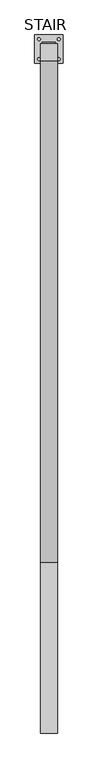
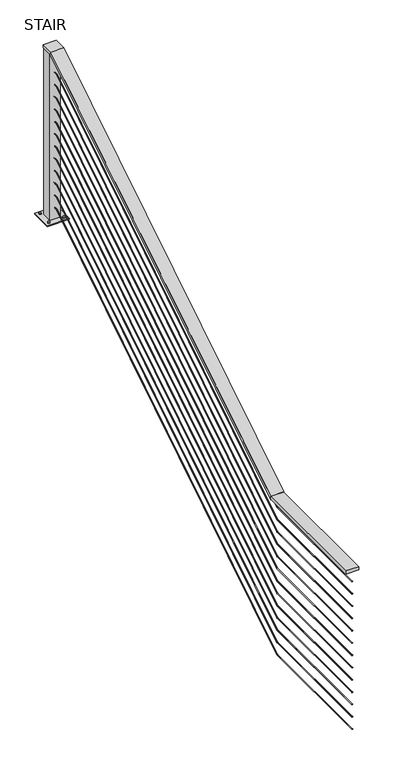
"""IFC4 building model written with IfcOpenShell, lengths in millimetres: railing geometry, STAIR."""

from ifc_helpers import new_model, si_unit, point, frame, frame_2d, origin, place, context, project, spatial, polyline, circle_curve, ellipse_curve, trimmed, segment, composite_curve, outline, extrude, faceted_brep, source, transform, mapped, element, save
from ifc_brep_helpers import plane_surface, cylinder_surface, advanced_brep


def stair_1ed1dee3(model_context):
    return source(origin(), model_context, "Body", "SolidModel", [
        faceted_brep([(26115.1620052, 2826.8043237, 2466.975), (26038.9620052, 2826.8043237, 2466.975), (26038.9620052, 2826.8043237, 2447.925), (26115.1620052, 2826.8043237, 2447.925), (26115.1620052, 3588.8043237, 2466.975), (26115.1620052, 3588.8043237, 2447.925), (26038.9620052, 3588.8043237, 2447.925), (26038.9620052, 3588.8043237, 2466.975)], [[[0, 1, 2, 3]], [[4, 5, 6, 7]], [[1, 0, 4, 7]], [[2, 1, 7, 6]], [[3, 2, 6, 5]], [[0, 3, 5, 4]]]),
        faceted_brep([(26115.1620052, 3588.8043237, 2468.6895104), (26038.9620052, 3588.8043237, 2468.6895104), (26038.9620052, 3588.8043237, 2446.2104896), (26115.1620052, 3588.8043237, 2446.2104896), (26115.1620052, 5821.2673274, 3867.15), (26038.9620052, 5821.2673274, 3867.15), (26038.9620052, 5826.7413199, 3848.1), (26115.1620052, 5826.7413199, 3848.1), (26115.1620052, 5898.8634079, 3867.15), (26115.1620052, 5898.8634079, 3848.1), (26038.9620052, 5898.8634079, 3848.1), (26038.9620052, 5898.8634079, 3867.15)], [[[0, 1, 2, 3]], [[1, 0, 4, 5]], [[2, 1, 5, 6]], [[3, 2, 6, 7]], [[0, 3, 7, 4]], [[8, 9, 10, 11]], [[5, 4, 8, 11]], [[6, 5, 11, 10]], [[7, 6, 10, 9]], [[4, 7, 9, 8]]]),
        advanced_brep(
        [(26074.6807552, 2826.8043237, 2388.39375), (26079.4432552, 2826.8043237, 2388.39375), (26074.6807552, 3588.8043237, 2388.39375), (26079.4432552, 3588.8043237, 2388.39375)],
        [
            (0, 1, circle_curve(frame((26077.0620052, 2826.8043237, 2388.39375), z_axis=(0.0, -1.0, 0.0), x_axis=(1.0, 0.0, 0.0)), 2.38125)),
            (1, 0, circle_curve(frame((26077.0620052, 2826.8043237, 2388.39375), z_axis=(0.0, -1.0, 0.0), x_axis=(1.0, 0.0, 0.0)), 2.38125)),
            (2, 3, circle_curve(frame((26077.0620052, 3588.8043237, 2388.39375), z_axis=(0.0, 1.0, 0.0), x_axis=(1.0, 0.0, 0.0)), 2.38125)),
            (3, 2, circle_curve(frame((26077.0620052, 3588.8043237, 2388.39375), z_axis=(0.0, 1.0, 0.0), x_axis=(1.0, 0.0, 0.0)), 2.38125)),
            (0, 2),
            (3, 1),
        ],
        [
            plane_surface(frame((26077.0620052, 2826.8043237, 2390.775), z_axis=(0.0, -1.0, 0.0), x_axis=(0.0, 0.0, 1.0))),
            plane_surface(frame((26077.0620052, 3588.8043237, 2390.775), z_axis=(0.0, 1.0, 0.0), x_axis=(0.0, 0.0, 1.0))),
            cylinder_surface(frame((26077.0620052, 2826.8043237, 2388.39375), z_axis=(0.0, -1.0, 0.0), x_axis=(1.0, 0.0, 0.0)), 2.38125),
        ],
        [
            (0, [[1, 2]]),
            (1, [[3, 4]]),
            (2, [[-1, 5, -4, 6]]),
            (2, [[-2, -6, -3, -5]]),
        ],
    ),
        advanced_brep(
        [(26074.6807552, 3588.8043237, 2387.9651224), (26079.4432552, 3588.8043237, 2387.9651224), (26074.6807552, 5824.6885727, 3788.56875), (26079.4432552, 5824.6885727, 3788.56875), (26074.6807552, 5898.8634079, 3788.56875), (26079.4432552, 5898.8634079, 3788.56875)],
        [
            (0, 1, ellipse_curve(frame((26077.0620052, 3588.8043237, 2387.9651224), z_axis=(0.0, -1.0, 0.0), x_axis=(0.0, 0.0, -1.0)), 2.8098776, 2.38125)),
            (1, 0, ellipse_curve(frame((26077.0620052, 3588.8043237, 2387.9651224), z_axis=(0.0, -1.0, 0.0), x_axis=(0.0, 0.0, -1.0)), 2.8098776, 2.38125)),
            (0, 2),
            (2, 3, ellipse_curve(frame((26077.0620052, 5824.6885727, 3788.56875), z_axis=(0.0, -0.9611079128273462, -0.2761730977134852), x_axis=(0.0, 0.27617309771348514, -0.9611079128273461)), 2.4776094, 2.38125)),
            (3, 1),
            (3, 2, ellipse_curve(frame((26077.0620052, 5824.6885727, 3788.56875), z_axis=(0.0, -0.9611079128273462, -0.2761730977134852), x_axis=(0.0, 0.27617309771348514, -0.9611079128273461)), 2.4776094, 2.38125)),
            (4, 5, circle_curve(frame((26077.0620052, 5898.8634079, 3788.56875), z_axis=(0.0, 1.0, 0.0), x_axis=(1.0, 0.0, 0.0)), 2.38125)),
            (5, 4, circle_curve(frame((26077.0620052, 5898.8634079, 3788.56875), z_axis=(0.0, 1.0, 0.0), x_axis=(1.0, 0.0, 0.0)), 2.38125)),
            (2, 4),
            (5, 3),
        ],
        [
            plane_surface(frame((26077.0620052, 3588.8043237, 2390.775), z_axis=(0.0, -1.0, 0.0), x_axis=(0.0, 0.0, 1.0))),
            cylinder_surface(frame((26077.0620052, 3590.0684443, 2388.7569934), z_axis=(0.0, -0.8474568401986755, -0.530864299044941), x_axis=(1.0, 0.0, 0.0)), 2.38125),
            plane_surface(frame((26077.0620052, 5898.8634079, 3790.95), z_axis=(0.0, 1.0, 0.0), x_axis=(0.0, 0.0, 1.0))),
            cylinder_surface(frame((26077.0620052, 5824.0043237, 3788.56875), z_axis=(0.0, -1.0, 0.0), x_axis=(1.0, 0.0, 0.0)), 2.38125),
        ],
        [
            (0, [[1, 2]]),
            (1, [[-1, 3, 4, 5]]),
            (1, [[-2, -5, 6, -3]]),
            (2, [[7, 8]]),
            (3, [[-4, 9, -8, 10]]),
            (3, [[-6, -10, -7, -9]]),
        ],
    ),
        advanced_brep(
        [(26074.6807552, 2826.8043237, 2312.19375), (26079.4432552, 2826.8043237, 2312.19375), (26074.6807552, 3588.8043237, 2312.19375), (26079.4432552, 3588.8043237, 2312.19375)],
        [
            (0, 1, circle_curve(frame((26077.0620052, 2826.8043237, 2312.19375), z_axis=(0.0, -1.0, 0.0), x_axis=(1.0, 0.0, 0.0)), 2.38125)),
            (1, 0, circle_curve(frame((26077.0620052, 2826.8043237, 2312.19375), z_axis=(0.0, -1.0, 0.0), x_axis=(1.0, 0.0, 0.0)), 2.38125)),
            (2, 3, circle_curve(frame((26077.0620052, 3588.8043237, 2312.19375), z_axis=(0.0, 1.0, 0.0), x_axis=(1.0, 0.0, 0.0)), 2.38125)),
            (3, 2, circle_curve(frame((26077.0620052, 3588.8043237, 2312.19375), z_axis=(0.0, 1.0, 0.0), x_axis=(1.0, 0.0, 0.0)), 2.38125)),
            (0, 2),
            (3, 1),
        ],
        [
            plane_surface(frame((26077.0620052, 2826.8043237, 2314.575), z_axis=(0.0, -1.0, 0.0), x_axis=(0.0, 0.0, 1.0))),
            plane_surface(frame((26077.0620052, 3588.8043237, 2314.575), z_axis=(0.0, 1.0, 0.0), x_axis=(0.0, 0.0, 1.0))),
            cylinder_surface(frame((26077.0620052, 2826.8043237, 2312.19375), z_axis=(0.0, -1.0, 0.0), x_axis=(1.0, 0.0, 0.0)), 2.38125),
        ],
        [
            (0, [[1, 2]]),
            (1, [[3, 4]]),
            (2, [[-1, 5, -4, 6]]),
            (2, [[-2, -6, -3, -5]]),
        ],
    ),
        advanced_brep(
        [(26074.6807552, 3588.8043237, 2311.7651224), (26079.4432552, 3588.8043237, 2311.7651224), (26074.6807552, 5824.6885727, 3712.36875), (26079.4432552, 5824.6885727, 3712.36875), (26074.6807552, 5898.8634079, 3712.36875), (26079.4432552, 5898.8634079, 3712.36875)],
        [
            (0, 1, ellipse_curve(frame((26077.0620052, 3588.8043237, 2311.7651224), z_axis=(0.0, -1.0, 0.0), x_axis=(0.0, 0.0, -1.0)), 2.8098776, 2.38125)),
            (1, 0, ellipse_curve(frame((26077.0620052, 3588.8043237, 2311.7651224), z_axis=(0.0, -1.0, 0.0), x_axis=(0.0, 0.0, -1.0)), 2.8098776, 2.38125)),
            (0, 2),
            (2, 3, ellipse_curve(frame((26077.0620052, 5824.6885727, 3712.36875), z_axis=(0.0, -0.9611079128273462, -0.2761730977134852), x_axis=(0.0, 0.27617309771348514, -0.9611079128273461)), 2.4776094, 2.38125)),
            (3, 1),
            (3, 2, ellipse_curve(frame((26077.0620052, 5824.6885727, 3712.36875), z_axis=(0.0, -0.9611079128273462, -0.2761730977134852), x_axis=(0.0, 0.27617309771348514, -0.9611079128273461)), 2.4776094, 2.38125)),
            (4, 5, circle_curve(frame((26077.0620052, 5898.8634079, 3712.36875), z_axis=(0.0, 1.0, 0.0), x_axis=(1.0, 0.0, 0.0)), 2.38125)),
            (5, 4, circle_curve(frame((26077.0620052, 5898.8634079, 3712.36875), z_axis=(0.0, 1.0, 0.0), x_axis=(1.0, 0.0, 0.0)), 2.38125)),
            (2, 4),
            (5, 3),
        ],
        [
            plane_surface(frame((26077.0620052, 3588.8043237, 2314.575), z_axis=(0.0, -1.0, 0.0), x_axis=(0.0, 0.0, 1.0))),
            cylinder_surface(frame((26077.0620052, 3590.0684443, 2312.5569934), z_axis=(0.0, -0.8474568401986755, -0.530864299044941), x_axis=(1.0, 0.0, 0.0)), 2.38125),
            plane_surface(frame((26077.0620052, 5898.8634079, 3714.75), z_axis=(0.0, 1.0, 0.0), x_axis=(0.0, 0.0, 1.0))),
            cylinder_surface(frame((26077.0620052, 5824.0043237, 3712.36875), z_axis=(0.0, -1.0, 0.0), x_axis=(1.0, 0.0, 0.0)), 2.38125),
        ],
        [
            (0, [[1, 2]]),
            (1, [[-1, 3, 4, 5]]),
            (1, [[-2, -5, 6, -3]]),
            (2, [[7, 8]]),
            (3, [[-4, 9, -8, 10]]),
            (3, [[-6, -10, -7, -9]]),
        ],
    ),
        advanced_brep(
        [(26074.6807552, 2826.8043237, 2235.99375), (26079.4432552, 2826.8043237, 2235.99375), (26074.6807552, 3588.8043237, 2235.99375), (26079.4432552, 3588.8043237, 2235.99375)],
        [
            (0, 1, circle_curve(frame((26077.0620052, 2826.8043237, 2235.99375), z_axis=(0.0, -1.0, 0.0), x_axis=(1.0, 0.0, 0.0)), 2.38125)),
            (1, 0, circle_curve(frame((26077.0620052, 2826.8043237, 2235.99375), z_axis=(0.0, -1.0, 0.0), x_axis=(1.0, 0.0, 0.0)), 2.38125)),
            (2, 3, circle_curve(frame((26077.0620052, 3588.8043237, 2235.99375), z_axis=(0.0, 1.0, 0.0), x_axis=(1.0, 0.0, 0.0)), 2.38125)),
            (3, 2, circle_curve(frame((26077.0620052, 3588.8043237, 2235.99375), z_axis=(0.0, 1.0, 0.0), x_axis=(1.0, 0.0, 0.0)), 2.38125)),
            (0, 2),
            (3, 1),
        ],
        [
            plane_surface(frame((26077.0620052, 2826.8043237, 2238.375), z_axis=(0.0, -1.0, 0.0), x_axis=(0.0, 0.0, 1.0))),
            plane_surface(frame((26077.0620052, 3588.8043237, 2238.375), z_axis=(0.0, 1.0, 0.0), x_axis=(0.0, 0.0, 1.0))),
            cylinder_surface(frame((26077.0620052, 2826.8043237, 2235.99375), z_axis=(0.0, -1.0, 0.0), x_axis=(1.0, 0.0, 0.0)), 2.38125),
        ],
        [
            (0, [[1, 2]]),
            (1, [[3, 4]]),
            (2, [[-1, 5, -4, 6]]),
            (2, [[-2, -6, -3, -5]]),
        ],
    ),
        advanced_brep(
        [(26074.6807552, 3588.8043237, 2235.5651224), (26079.4432552, 3588.8043237, 2235.5651224), (26074.6807552, 5824.6885727, 3636.16875), (26079.4432552, 5824.6885727, 3636.16875), (26074.6807552, 5898.8634079, 3636.16875), (26079.4432552, 5898.8634079, 3636.16875)],
        [
            (0, 1, ellipse_curve(frame((26077.0620052, 3588.8043237, 2235.5651224), z_axis=(0.0, -1.0, 0.0), x_axis=(0.0, 0.0, -1.0)), 2.8098776, 2.38125)),
            (1, 0, ellipse_curve(frame((26077.0620052, 3588.8043237, 2235.5651224), z_axis=(0.0, -1.0, 0.0), x_axis=(0.0, 0.0, -1.0)), 2.8098776, 2.38125)),
            (0, 2),
            (2, 3, ellipse_curve(frame((26077.0620052, 5824.6885727, 3636.16875), z_axis=(0.0, -0.9611079128273462, -0.2761730977134852), x_axis=(0.0, 0.27617309771348514, -0.9611079128273461)), 2.4776094, 2.38125)),
            (3, 1),
            (3, 2, ellipse_curve(frame((26077.0620052, 5824.6885727, 3636.16875), z_axis=(0.0, -0.9611079128273462, -0.2761730977134852), x_axis=(0.0, 0.27617309771348514, -0.9611079128273461)), 2.4776094, 2.38125)),
            (4, 5, circle_curve(frame((26077.0620052, 5898.8634079, 3636.16875), z_axis=(0.0, 1.0, 0.0), x_axis=(1.0, 0.0, 0.0)), 2.38125)),
            (5, 4, circle_curve(frame((26077.0620052, 5898.8634079, 3636.16875), z_axis=(0.0, 1.0, 0.0), x_axis=(1.0, 0.0, 0.0)), 2.38125)),
            (2, 4),
            (5, 3),
        ],
        [
            plane_surface(frame((26077.0620052, 3588.8043237, 2238.375), z_axis=(0.0, -1.0, 0.0), x_axis=(0.0, 0.0, 1.0))),
            cylinder_surface(frame((26077.0620052, 3590.0684443, 2236.3569934), z_axis=(0.0, -0.8474568401986755, -0.530864299044941), x_axis=(1.0, 0.0, 0.0)), 2.38125),
            plane_surface(frame((26077.0620052, 5898.8634079, 3638.55), z_axis=(0.0, 1.0, 0.0), x_axis=(0.0, 0.0, 1.0))),
            cylinder_surface(frame((26077.0620052, 5824.0043237, 3636.16875), z_axis=(0.0, -1.0, 0.0), x_axis=(1.0, 0.0, 0.0)), 2.38125),
        ],
        [
            (0, [[1, 2]]),
            (1, [[-1, 3, 4, 5]]),
            (1, [[-2, -5, 6, -3]]),
            (2, [[7, 8]]),
            (3, [[-4, 9, -8, 10]]),
            (3, [[-6, -10, -7, -9]]),
        ],
    ),
        advanced_brep(
        [(26074.6807552, 2826.8043237, 2159.79375), (26079.4432552, 2826.8043237, 2159.79375), (26074.6807552, 3588.8043237, 2159.79375), (26079.4432552, 3588.8043237, 2159.79375)],
        [
            (0, 1, circle_curve(frame((26077.0620052, 2826.8043237, 2159.79375), z_axis=(0.0, -1.0, 0.0), x_axis=(1.0, 0.0, 0.0)), 2.38125)),
            (1, 0, circle_curve(frame((26077.0620052, 2826.8043237, 2159.79375), z_axis=(0.0, -1.0, 0.0), x_axis=(1.0, 0.0, 0.0)), 2.38125)),
            (2, 3, circle_curve(frame((26077.0620052, 3588.8043237, 2159.79375), z_axis=(0.0, 1.0, 0.0), x_axis=(1.0, 0.0, 0.0)), 2.38125)),
            (3, 2, circle_curve(frame((26077.0620052, 3588.8043237, 2159.79375), z_axis=(0.0, 1.0, 0.0), x_axis=(1.0, 0.0, 0.0)), 2.38125)),
            (0, 2),
            (3, 1),
        ],
        [
            plane_surface(frame((26077.0620052, 2826.8043237, 2162.175), z_axis=(0.0, -1.0, 0.0), x_axis=(0.0, 0.0, 1.0))),
            plane_surface(frame((26077.0620052, 3588.8043237, 2162.175), z_axis=(0.0, 1.0, 0.0), x_axis=(0.0, 0.0, 1.0))),
            cylinder_surface(frame((26077.0620052, 2826.8043237, 2159.79375), z_axis=(0.0, -1.0, 0.0), x_axis=(1.0, 0.0, 0.0)), 2.38125),
        ],
        [
            (0, [[1, 2]]),
            (1, [[3, 4]]),
            (2, [[-1, 5, -4, 6]]),
            (2, [[-2, -6, -3, -5]]),
        ],
    ),
        advanced_brep(
        [(26074.6807552, 3588.8043237, 2159.3651224), (26079.4432552, 3588.8043237, 2159.3651224), (26074.6807552, 5824.6885727, 3559.96875), (26079.4432552, 5824.6885727, 3559.96875), (26074.6807552, 5898.8634079, 3559.96875), (26079.4432552, 5898.8634079, 3559.96875)],
        [
            (0, 1, ellipse_curve(frame((26077.0620052, 3588.8043237, 2159.3651224), z_axis=(0.0, -1.0, 0.0), x_axis=(0.0, 0.0, -1.0)), 2.8098776, 2.38125)),
            (1, 0, ellipse_curve(frame((26077.0620052, 3588.8043237, 2159.3651224), z_axis=(0.0, -1.0, 0.0), x_axis=(0.0, 0.0, -1.0)), 2.8098776, 2.38125)),
            (0, 2),
            (2, 3, ellipse_curve(frame((26077.0620052, 5824.6885727, 3559.96875), z_axis=(0.0, -0.9611079128273462, -0.2761730977134852), x_axis=(0.0, 0.27617309771348514, -0.9611079128273461)), 2.4776094, 2.38125)),
            (3, 1),
            (3, 2, ellipse_curve(frame((26077.0620052, 5824.6885727, 3559.96875), z_axis=(0.0, -0.9611079128273462, -0.2761730977134852), x_axis=(0.0, 0.27617309771348514, -0.9611079128273461)), 2.4776094, 2.38125)),
            (4, 5, circle_curve(frame((26077.0620052, 5898.8634079, 3559.96875), z_axis=(0.0, 1.0, 0.0), x_axis=(1.0, 0.0, 0.0)), 2.38125)),
            (5, 4, circle_curve(frame((26077.0620052, 5898.8634079, 3559.96875), z_axis=(0.0, 1.0, 0.0), x_axis=(1.0, 0.0, 0.0)), 2.38125)),
            (2, 4),
            (5, 3),
        ],
        [
            plane_surface(frame((26077.0620052, 3588.8043237, 2162.175), z_axis=(0.0, -1.0, 0.0), x_axis=(0.0, 0.0, 1.0))),
            cylinder_surface(frame((26077.0620052, 3590.0684443, 2160.1569934), z_axis=(0.0, -0.8474568401986755, -0.530864299044941), x_axis=(1.0, 0.0, 0.0)), 2.38125),
            plane_surface(frame((26077.0620052, 5898.8634079, 3562.35), z_axis=(0.0, 1.0, 0.0), x_axis=(0.0, 0.0, 1.0))),
            cylinder_surface(frame((26077.0620052, 5824.0043237, 3559.96875), z_axis=(0.0, -1.0, 0.0), x_axis=(1.0, 0.0, 0.0)), 2.38125),
        ],
        [
            (0, [[1, 2]]),
            (1, [[-1, 3, 4, 5]]),
            (1, [[-2, -5, 6, -3]]),
            (2, [[7, 8]]),
            (3, [[-4, 9, -8, 10]]),
            (3, [[-6, -10, -7, -9]]),
        ],
    ),
        advanced_brep(
        [(26074.6807552, 2826.8043237, 2083.59375), (26079.4432552, 2826.8043237, 2083.59375), (26074.6807552, 3588.8043237, 2083.59375), (26079.4432552, 3588.8043237, 2083.59375)],
        [
            (0, 1, circle_curve(frame((26077.0620052, 2826.8043237, 2083.59375), z_axis=(0.0, -1.0, 0.0), x_axis=(1.0, 0.0, 0.0)), 2.38125)),
            (1, 0, circle_curve(frame((26077.0620052, 2826.8043237, 2083.59375), z_axis=(0.0, -1.0, 0.0), x_axis=(1.0, 0.0, 0.0)), 2.38125)),
            (2, 3, circle_curve(frame((26077.0620052, 3588.8043237, 2083.59375), z_axis=(0.0, 1.0, 0.0), x_axis=(1.0, 0.0, 0.0)), 2.38125)),
            (3, 2, circle_curve(frame((26077.0620052, 3588.8043237, 2083.59375), z_axis=(0.0, 1.0, 0.0), x_axis=(1.0, 0.0, 0.0)), 2.38125)),
            (0, 2),
            (3, 1),
        ],
        [
            plane_surface(frame((26077.0620052, 2826.8043237, 2085.975), z_axis=(0.0, -1.0, 0.0), x_axis=(0.0, 0.0, 1.0))),
            plane_surface(frame((26077.0620052, 3588.8043237, 2085.975), z_axis=(0.0, 1.0, 0.0), x_axis=(0.0, 0.0, 1.0))),
            cylinder_surface(frame((26077.0620052, 2826.8043237, 2083.59375), z_axis=(0.0, -1.0, 0.0), x_axis=(1.0, 0.0, 0.0)), 2.38125),
        ],
        [
            (0, [[1, 2]]),
            (1, [[3, 4]]),
            (2, [[-1, 5, -4, 6]]),
            (2, [[-2, -6, -3, -5]]),
        ],
    ),
        advanced_brep(
        [(26074.6807552, 3588.8043237, 2083.1651224), (26079.4432552, 3588.8043237, 2083.1651224), (26074.6807552, 5824.6885727, 3483.76875), (26079.4432552, 5824.6885727, 3483.76875), (26074.6807552, 5898.8634079, 3483.76875), (26079.4432552, 5898.8634079, 3483.76875)],
        [
            (0, 1, ellipse_curve(frame((26077.0620052, 3588.8043237, 2083.1651224), z_axis=(0.0, -1.0, 0.0), x_axis=(0.0, 0.0, -1.0)), 2.8098776, 2.38125)),
            (1, 0, ellipse_curve(frame((26077.0620052, 3588.8043237, 2083.1651224), z_axis=(0.0, -1.0, 0.0), x_axis=(0.0, 0.0, -1.0)), 2.8098776, 2.38125)),
            (0, 2),
            (2, 3, ellipse_curve(frame((26077.0620052, 5824.6885727, 3483.76875), z_axis=(0.0, -0.9611079128273462, -0.2761730977134852), x_axis=(0.0, 0.27617309771348514, -0.9611079128273461)), 2.4776094, 2.38125)),
            (3, 1),
            (3, 2, ellipse_curve(frame((26077.0620052, 5824.6885727, 3483.76875), z_axis=(0.0, -0.9611079128273462, -0.2761730977134852), x_axis=(0.0, 0.27617309771348514, -0.9611079128273461)), 2.4776094, 2.38125)),
            (4, 5, circle_curve(frame((26077.0620052, 5898.8634079, 3483.76875), z_axis=(0.0, 1.0, 0.0), x_axis=(1.0, 0.0, 0.0)), 2.38125)),
            (5, 4, circle_curve(frame((26077.0620052, 5898.8634079, 3483.76875), z_axis=(0.0, 1.0, 0.0), x_axis=(1.0, 0.0, 0.0)), 2.38125)),
            (2, 4),
            (5, 3),
        ],
        [
            plane_surface(frame((26077.0620052, 3588.8043237, 2085.975), z_axis=(0.0, -1.0, 0.0), x_axis=(0.0, 0.0, 1.0))),
            cylinder_surface(frame((26077.0620052, 3590.0684443, 2083.9569934), z_axis=(0.0, -0.8474568401986755, -0.530864299044941), x_axis=(1.0, 0.0, 0.0)), 2.38125),
            plane_surface(frame((26077.0620052, 5898.8634079, 3486.15), z_axis=(0.0, 1.0, 0.0), x_axis=(0.0, 0.0, 1.0))),
            cylinder_surface(frame((26077.0620052, 5824.0043237, 3483.76875), z_axis=(0.0, -1.0, 0.0), x_axis=(1.0, 0.0, 0.0)), 2.38125),
        ],
        [
            (0, [[1, 2]]),
            (1, [[-1, 3, 4, 5]]),
            (1, [[-2, -5, 6, -3]]),
            (2, [[7, 8]]),
            (3, [[-4, 9, -8, 10]]),
            (3, [[-6, -10, -7, -9]]),
        ],
    ),
        advanced_brep(
        [(26074.6807552, 2826.8043237, 2007.39375), (26079.4432552, 2826.8043237, 2007.39375), (26074.6807552, 3588.8043237, 2007.39375), (26079.4432552, 3588.8043237, 2007.39375)],
        [
            (0, 1, circle_curve(frame((26077.0620052, 2826.8043237, 2007.39375), z_axis=(0.0, -1.0, 0.0), x_axis=(1.0, 0.0, 0.0)), 2.38125)),
            (1, 0, circle_curve(frame((26077.0620052, 2826.8043237, 2007.39375), z_axis=(0.0, -1.0, 0.0), x_axis=(1.0, 0.0, 0.0)), 2.38125)),
            (2, 3, circle_curve(frame((26077.0620052, 3588.8043237, 2007.39375), z_axis=(0.0, 1.0, 0.0), x_axis=(1.0, 0.0, 0.0)), 2.38125)),
            (3, 2, circle_curve(frame((26077.0620052, 3588.8043237, 2007.39375), z_axis=(0.0, 1.0, 0.0), x_axis=(1.0, 0.0, 0.0)), 2.38125)),
            (0, 2),
            (3, 1),
        ],
        [
            plane_surface(frame((26077.0620052, 2826.8043237, 2009.775), z_axis=(0.0, -1.0, 0.0), x_axis=(0.0, 0.0, 1.0))),
            plane_surface(frame((26077.0620052, 3588.8043237, 2009.775), z_axis=(0.0, 1.0, 0.0), x_axis=(0.0, 0.0, 1.0))),
            cylinder_surface(frame((26077.0620052, 2826.8043237, 2007.39375), z_axis=(0.0, -1.0, 0.0), x_axis=(1.0, 0.0, 0.0)), 2.38125),
        ],
        [
            (0, [[1, 2]]),
            (1, [[3, 4]]),
            (2, [[-1, 5, -4, 6]]),
            (2, [[-2, -6, -3, -5]]),
        ],
    ),
        advanced_brep(
        [(26074.6807552, 3588.8043237, 2006.9651224), (26079.4432552, 3588.8043237, 2006.9651224), (26074.6807552, 5824.6885727, 3407.56875), (26079.4432552, 5824.6885727, 3407.56875), (26074.6807552, 5898.8634079, 3407.56875), (26079.4432552, 5898.8634079, 3407.56875)],
        [
            (0, 1, ellipse_curve(frame((26077.0620052, 3588.8043237, 2006.9651224), z_axis=(0.0, -1.0, 0.0), x_axis=(0.0, 0.0, -1.0)), 2.8098776, 2.38125)),
            (1, 0, ellipse_curve(frame((26077.0620052, 3588.8043237, 2006.9651224), z_axis=(0.0, -1.0, 0.0), x_axis=(0.0, 0.0, -1.0)), 2.8098776, 2.38125)),
            (0, 2),
            (2, 3, ellipse_curve(frame((26077.0620052, 5824.6885727, 3407.56875), z_axis=(0.0, -0.9611079128273462, -0.2761730977134852), x_axis=(0.0, 0.27617309771348514, -0.9611079128273461)), 2.4776094, 2.38125)),
            (3, 1),
            (3, 2, ellipse_curve(frame((26077.0620052, 5824.6885727, 3407.56875), z_axis=(0.0, -0.9611079128273462, -0.2761730977134852), x_axis=(0.0, 0.27617309771348514, -0.9611079128273461)), 2.4776094, 2.38125)),
            (4, 5, circle_curve(frame((26077.0620052, 5898.8634079, 3407.56875), z_axis=(0.0, 1.0, 0.0), x_axis=(1.0, 0.0, 0.0)), 2.38125)),
            (5, 4, circle_curve(frame((26077.0620052, 5898.8634079, 3407.56875), z_axis=(0.0, 1.0, 0.0), x_axis=(1.0, 0.0, 0.0)), 2.38125)),
            (2, 4),
            (5, 3),
        ],
        [
            plane_surface(frame((26077.0620052, 3588.8043237, 2009.775), z_axis=(0.0, -1.0, 0.0), x_axis=(0.0, 0.0, 1.0))),
            cylinder_surface(frame((26077.0620052, 3590.0684443, 2007.7569934), z_axis=(0.0, -0.8474568401986755, -0.530864299044941), x_axis=(1.0, 0.0, 0.0)), 2.38125),
            plane_surface(frame((26077.0620052, 5898.8634079, 3409.95), z_axis=(0.0, 1.0, 0.0), x_axis=(0.0, 0.0, 1.0))),
            cylinder_surface(frame((26077.0620052, 5824.0043237, 3407.56875), z_axis=(0.0, -1.0, 0.0), x_axis=(1.0, 0.0, 0.0)), 2.38125),
        ],
        [
            (0, [[1, 2]]),
            (1, [[-1, 3, 4, 5]]),
            (1, [[-2, -5, 6, -3]]),
            (2, [[7, 8]]),
            (3, [[-4, 9, -8, 10]]),
            (3, [[-6, -10, -7, -9]]),
        ],
    ),
        advanced_brep(
        [(26074.6807552, 2826.8043237, 1931.19375), (26079.4432552, 2826.8043237, 1931.19375), (26074.6807552, 3588.8043237, 1931.19375), (26079.4432552, 3588.8043237, 1931.19375)],
        [
            (0, 1, circle_curve(frame((26077.0620052, 2826.8043237, 1931.19375), z_axis=(0.0, -1.0, 0.0), x_axis=(1.0, 0.0, 0.0)), 2.38125)),
            (1, 0, circle_curve(frame((26077.0620052, 2826.8043237, 1931.19375), z_axis=(0.0, -1.0, 0.0), x_axis=(1.0, 0.0, 0.0)), 2.38125)),
            (2, 3, circle_curve(frame((26077.0620052, 3588.8043237, 1931.19375), z_axis=(0.0, 1.0, 0.0), x_axis=(1.0, 0.0, 0.0)), 2.38125)),
            (3, 2, circle_curve(frame((26077.0620052, 3588.8043237, 1931.19375), z_axis=(0.0, 1.0, 0.0), x_axis=(1.0, 0.0, 0.0)), 2.38125)),
            (0, 2),
            (3, 1),
        ],
        [
            plane_surface(frame((26077.0620052, 2826.8043237, 1933.575), z_axis=(0.0, -1.0, 0.0), x_axis=(0.0, 0.0, 1.0))),
            plane_surface(frame((26077.0620052, 3588.8043237, 1933.575), z_axis=(0.0, 1.0, 0.0), x_axis=(0.0, 0.0, 1.0))),
            cylinder_surface(frame((26077.0620052, 2826.8043237, 1931.19375), z_axis=(0.0, -1.0, 0.0), x_axis=(1.0, 0.0, 0.0)), 2.38125),
        ],
        [
            (0, [[1, 2]]),
            (1, [[3, 4]]),
            (2, [[-1, 5, -4, 6]]),
            (2, [[-2, -6, -3, -5]]),
        ],
    ),
        advanced_brep(
        [(26074.6807552, 3588.8043237, 1930.7651224), (26079.4432552, 3588.8043237, 1930.7651224), (26074.6807552, 5824.6885727, 3331.36875), (26079.4432552, 5824.6885727, 3331.36875), (26074.6807552, 5898.8634079, 3331.36875), (26079.4432552, 5898.8634079, 3331.36875)],
        [
            (0, 1, ellipse_curve(frame((26077.0620052, 3588.8043237, 1930.7651224), z_axis=(0.0, -1.0, 0.0), x_axis=(0.0, 0.0, -1.0)), 2.8098776, 2.38125)),
            (1, 0, ellipse_curve(frame((26077.0620052, 3588.8043237, 1930.7651224), z_axis=(0.0, -1.0, 0.0), x_axis=(0.0, 0.0, -1.0)), 2.8098776, 2.38125)),
            (0, 2),
            (2, 3, ellipse_curve(frame((26077.0620052, 5824.6885727, 3331.36875), z_axis=(0.0, -0.9611079128273462, -0.2761730977134852), x_axis=(0.0, 0.27617309771348514, -0.9611079128273461)), 2.4776094, 2.38125)),
            (3, 1),
            (3, 2, ellipse_curve(frame((26077.0620052, 5824.6885727, 3331.36875), z_axis=(0.0, -0.9611079128273462, -0.2761730977134852), x_axis=(0.0, 0.27617309771348514, -0.9611079128273461)), 2.4776094, 2.38125)),
            (4, 5, circle_curve(frame((26077.0620052, 5898.8634079, 3331.36875), z_axis=(0.0, 1.0, 0.0), x_axis=(1.0, 0.0, 0.0)), 2.38125)),
            (5, 4, circle_curve(frame((26077.0620052, 5898.8634079, 3331.36875), z_axis=(0.0, 1.0, 0.0), x_axis=(1.0, 0.0, 0.0)), 2.38125)),
            (2, 4),
            (5, 3),
        ],
        [
            plane_surface(frame((26077.0620052, 3588.8043237, 1933.575), z_axis=(0.0, -1.0, 0.0), x_axis=(0.0, 0.0, 1.0))),
            cylinder_surface(frame((26077.0620052, 3590.0684443, 1931.5569934), z_axis=(0.0, -0.8474568401986755, -0.530864299044941), x_axis=(1.0, 0.0, 0.0)), 2.38125),
            plane_surface(frame((26077.0620052, 5898.8634079, 3333.75), z_axis=(0.0, 1.0, 0.0), x_axis=(0.0, 0.0, 1.0))),
            cylinder_surface(frame((26077.0620052, 5824.0043237, 3331.36875), z_axis=(0.0, -1.0, 0.0), x_axis=(1.0, 0.0, 0.0)), 2.38125),
        ],
        [
            (0, [[1, 2]]),
            (1, [[-1, 3, 4, 5]]),
            (1, [[-2, -5, 6, -3]]),
            (2, [[7, 8]]),
            (3, [[-4, 9, -8, 10]]),
            (3, [[-6, -10, -7, -9]]),
        ],
    ),
        advanced_brep(
        [(26074.6807552, 2826.8043237, 1854.99375), (26079.4432552, 2826.8043237, 1854.99375), (26074.6807552, 3588.8043237, 1854.99375), (26079.4432552, 3588.8043237, 1854.99375)],
        [
            (0, 1, circle_curve(frame((26077.0620052, 2826.8043237, 1854.99375), z_axis=(0.0, -1.0, 0.0), x_axis=(1.0, 0.0, 0.0)), 2.38125)),
            (1, 0, circle_curve(frame((26077.0620052, 2826.8043237, 1854.99375), z_axis=(0.0, -1.0, 0.0), x_axis=(1.0, 0.0, 0.0)), 2.38125)),
            (2, 3, circle_curve(frame((26077.0620052, 3588.8043237, 1854.99375), z_axis=(0.0, 1.0, 0.0), x_axis=(1.0, 0.0, 0.0)), 2.38125)),
            (3, 2, circle_curve(frame((26077.0620052, 3588.8043237, 1854.99375), z_axis=(0.0, 1.0, 0.0), x_axis=(1.0, 0.0, 0.0)), 2.38125)),
            (0, 2),
            (3, 1),
        ],
        [
            plane_surface(frame((26077.0620052, 2826.8043237, 1857.375), z_axis=(0.0, -1.0, 0.0), x_axis=(0.0, 0.0, 1.0))),
            plane_surface(frame((26077.0620052, 3588.8043237, 1857.375), z_axis=(0.0, 1.0, 0.0), x_axis=(0.0, 0.0, 1.0))),
            cylinder_surface(frame((26077.0620052, 2826.8043237, 1854.99375), z_axis=(0.0, -1.0, 0.0), x_axis=(1.0, 0.0, 0.0)), 2.38125),
        ],
        [
            (0, [[1, 2]]),
            (1, [[3, 4]]),
            (2, [[-1, 5, -4, 6]]),
            (2, [[-2, -6, -3, -5]]),
        ],
    ),
        advanced_brep(
        [(26074.6807552, 3588.8043237, 1854.5651224), (26079.4432552, 3588.8043237, 1854.5651224), (26074.6807552, 5824.6885727, 3255.16875), (26079.4432552, 5824.6885727, 3255.16875), (26074.6807552, 5898.8634079, 3255.16875), (26079.4432552, 5898.8634079, 3255.16875)],
        [
            (0, 1, ellipse_curve(frame((26077.0620052, 3588.8043237, 1854.5651224), z_axis=(0.0, -1.0, 0.0), x_axis=(0.0, 0.0, -1.0)), 2.8098776, 2.38125)),
            (1, 0, ellipse_curve(frame((26077.0620052, 3588.8043237, 1854.5651224), z_axis=(0.0, -1.0, 0.0), x_axis=(0.0, 0.0, -1.0)), 2.8098776, 2.38125)),
            (0, 2),
            (2, 3, ellipse_curve(frame((26077.0620052, 5824.6885727, 3255.16875), z_axis=(0.0, -0.9611079128273462, -0.2761730977134852), x_axis=(0.0, 0.27617309771348514, -0.9611079128273461)), 2.4776094, 2.38125)),
            (3, 1),
            (3, 2, ellipse_curve(frame((26077.0620052, 5824.6885727, 3255.16875), z_axis=(0.0, -0.9611079128273462, -0.2761730977134852), x_axis=(0.0, 0.27617309771348514, -0.9611079128273461)), 2.4776094, 2.38125)),
            (4, 5, circle_curve(frame((26077.0620052, 5898.8634079, 3255.16875), z_axis=(0.0, 1.0, 0.0), x_axis=(1.0, 0.0, 0.0)), 2.38125)),
            (5, 4, circle_curve(frame((26077.0620052, 5898.8634079, 3255.16875), z_axis=(0.0, 1.0, 0.0), x_axis=(1.0, 0.0, 0.0)), 2.38125)),
            (2, 4),
            (5, 3),
        ],
        [
            plane_surface(frame((26077.0620052, 3588.8043237, 1857.375), z_axis=(0.0, -1.0, 0.0), x_axis=(0.0, 0.0, 1.0))),
            cylinder_surface(frame((26077.0620052, 3590.0684443, 1855.3569934), z_axis=(0.0, -0.8474568401986755, -0.530864299044941), x_axis=(1.0, 0.0, 0.0)), 2.38125),
            plane_surface(frame((26077.0620052, 5898.8634079, 3257.55), z_axis=(0.0, 1.0, 0.0), x_axis=(0.0, 0.0, 1.0))),
            cylinder_surface(frame((26077.0620052, 5824.0043237, 3255.16875), z_axis=(0.0, -1.0, 0.0), x_axis=(1.0, 0.0, 0.0)), 2.38125),
        ],
        [
            (0, [[1, 2]]),
            (1, [[-1, 3, 4, 5]]),
            (1, [[-2, -5, 6, -3]]),
            (2, [[7, 8]]),
            (3, [[-4, 9, -8, 10]]),
            (3, [[-6, -10, -7, -9]]),
        ],
    ),
        advanced_brep(
        [(26074.6807552, 2826.8043237, 1778.79375), (26079.4432552, 2826.8043237, 1778.79375), (26074.6807552, 3588.8043237, 1778.79375), (26079.4432552, 3588.8043237, 1778.79375)],
        [
            (0, 1, circle_curve(frame((26077.0620052, 2826.8043237, 1778.79375), z_axis=(0.0, -1.0, 0.0), x_axis=(1.0, 0.0, 0.0)), 2.38125)),
            (1, 0, circle_curve(frame((26077.0620052, 2826.8043237, 1778.79375), z_axis=(0.0, -1.0, 0.0), x_axis=(1.0, 0.0, 0.0)), 2.38125)),
            (2, 3, circle_curve(frame((26077.0620052, 3588.8043237, 1778.79375), z_axis=(0.0, 1.0, 0.0), x_axis=(1.0, 0.0, 0.0)), 2.38125)),
            (3, 2, circle_curve(frame((26077.0620052, 3588.8043237, 1778.79375), z_axis=(0.0, 1.0, 0.0), x_axis=(1.0, 0.0, 0.0)), 2.38125)),
            (0, 2),
            (3, 1),
        ],
        [
            plane_surface(frame((26077.0620052, 2826.8043237, 1781.175), z_axis=(0.0, -1.0, 0.0), x_axis=(0.0, 0.0, 1.0))),
            plane_surface(frame((26077.0620052, 3588.8043237, 1781.175), z_axis=(0.0, 1.0, 0.0), x_axis=(0.0, 0.0, 1.0))),
            cylinder_surface(frame((26077.0620052, 2826.8043237, 1778.79375), z_axis=(0.0, -1.0, 0.0), x_axis=(1.0, 0.0, 0.0)), 2.38125),
        ],
        [
            (0, [[1, 2]]),
            (1, [[3, 4]]),
            (2, [[-1, 5, -4, 6]]),
            (2, [[-2, -6, -3, -5]]),
        ],
    ),
        advanced_brep(
        [(26074.6807552, 3588.8043237, 1778.3651224), (26079.4432552, 3588.8043237, 1778.3651224), (26074.6807552, 5824.6885727, 3178.96875), (26079.4432552, 5824.6885727, 3178.96875), (26074.6807552, 5898.8634079, 3178.96875), (26079.4432552, 5898.8634079, 3178.96875)],
        [
            (0, 1, ellipse_curve(frame((26077.0620052, 3588.8043237, 1778.3651224), z_axis=(0.0, -1.0, 0.0), x_axis=(0.0, 0.0, -1.0)), 2.8098776, 2.38125)),
            (1, 0, ellipse_curve(frame((26077.0620052, 3588.8043237, 1778.3651224), z_axis=(0.0, -1.0, 0.0), x_axis=(0.0, 0.0, -1.0)), 2.8098776, 2.38125)),
            (0, 2),
            (2, 3, ellipse_curve(frame((26077.0620052, 5824.6885727, 3178.96875), z_axis=(0.0, -0.9611079128273462, -0.2761730977134852), x_axis=(0.0, 0.27617309771348514, -0.9611079128273461)), 2.4776094, 2.38125)),
            (3, 1),
            (3, 2, ellipse_curve(frame((26077.0620052, 5824.6885727, 3178.96875), z_axis=(0.0, -0.9611079128273462, -0.2761730977134852), x_axis=(0.0, 0.27617309771348514, -0.9611079128273461)), 2.4776094, 2.38125)),
            (4, 5, circle_curve(frame((26077.0620052, 5898.8634079, 3178.96875), z_axis=(0.0, 1.0, 0.0), x_axis=(1.0, 0.0, 0.0)), 2.38125)),
            (5, 4, circle_curve(frame((26077.0620052, 5898.8634079, 3178.96875), z_axis=(0.0, 1.0, 0.0), x_axis=(1.0, 0.0, 0.0)), 2.38125)),
            (2, 4),
            (5, 3),
        ],
        [
            plane_surface(frame((26077.0620052, 3588.8043237, 1781.175), z_axis=(0.0, -1.0, 0.0), x_axis=(0.0, 0.0, 1.0))),
            cylinder_surface(frame((26077.0620052, 3590.0684443, 1779.1569934), z_axis=(0.0, -0.8474568401986755, -0.530864299044941), x_axis=(1.0, 0.0, 0.0)), 2.38125),
            plane_surface(frame((26077.0620052, 5898.8634079, 3181.35), z_axis=(0.0, 1.0, 0.0), x_axis=(0.0, 0.0, 1.0))),
            cylinder_surface(frame((26077.0620052, 5824.0043237, 3178.96875), z_axis=(0.0, -1.0, 0.0), x_axis=(1.0, 0.0, 0.0)), 2.38125),
        ],
        [
            (0, [[1, 2]]),
            (1, [[-1, 3, 4, 5]]),
            (1, [[-2, -5, 6, -3]]),
            (2, [[7, 8]]),
            (3, [[-4, 9, -8, 10]]),
            (3, [[-6, -10, -7, -9]]),
        ],
    ),
        advanced_brep(
        [(26074.6807552, 2826.8043237, 1702.59375), (26079.4432552, 2826.8043237, 1702.59375), (26074.6807552, 3588.8043237, 1702.59375), (26079.4432552, 3588.8043237, 1702.59375)],
        [
            (0, 1, circle_curve(frame((26077.0620052, 2826.8043237, 1702.59375), z_axis=(0.0, -1.0, 0.0), x_axis=(1.0, 0.0, 0.0)), 2.38125)),
            (1, 0, circle_curve(frame((26077.0620052, 2826.8043237, 1702.59375), z_axis=(0.0, -1.0, 0.0), x_axis=(1.0, 0.0, 0.0)), 2.38125)),
            (2, 3, circle_curve(frame((26077.0620052, 3588.8043237, 1702.59375), z_axis=(0.0, 1.0, 0.0), x_axis=(1.0, 0.0, 0.0)), 2.38125)),
            (3, 2, circle_curve(frame((26077.0620052, 3588.8043237, 1702.59375), z_axis=(0.0, 1.0, 0.0), x_axis=(1.0, 0.0, 0.0)), 2.38125)),
            (0, 2),
            (3, 1),
        ],
        [
            plane_surface(frame((26077.0620052, 2826.8043237, 1704.975), z_axis=(0.0, -1.0, 0.0), x_axis=(0.0, 0.0, 1.0))),
            plane_surface(frame((26077.0620052, 3588.8043237, 1704.975), z_axis=(0.0, 1.0, 0.0), x_axis=(0.0, 0.0, 1.0))),
            cylinder_surface(frame((26077.0620052, 2826.8043237, 1702.59375), z_axis=(0.0, -1.0, 0.0), x_axis=(1.0, 0.0, 0.0)), 2.38125),
        ],
        [
            (0, [[1, 2]]),
            (1, [[3, 4]]),
            (2, [[-1, 5, -4, 6]]),
            (2, [[-2, -6, -3, -5]]),
        ],
    ),
        advanced_brep(
        [(26074.6807552, 3588.8043237, 1702.1651224), (26079.4432552, 3588.8043237, 1702.1651224), (26074.6807552, 5824.6885727, 3102.76875), (26079.4432552, 5824.6885727, 3102.76875), (26074.6807552, 5898.8634079, 3102.76875), (26079.4432552, 5898.8634079, 3102.76875)],
        [
            (0, 1, ellipse_curve(frame((26077.0620052, 3588.8043237, 1702.1651224), z_axis=(0.0, -1.0, 0.0), x_axis=(0.0, 0.0, -1.0)), 2.8098776, 2.38125)),
            (1, 0, ellipse_curve(frame((26077.0620052, 3588.8043237, 1702.1651224), z_axis=(0.0, -1.0, 0.0), x_axis=(0.0, 0.0, -1.0)), 2.8098776, 2.38125)),
            (0, 2),
            (2, 3, ellipse_curve(frame((26077.0620052, 5824.6885727, 3102.76875), z_axis=(0.0, -0.9611079128273462, -0.2761730977134852), x_axis=(0.0, 0.27617309771348514, -0.9611079128273461)), 2.4776094, 2.38125)),
            (3, 1),
            (3, 2, ellipse_curve(frame((26077.0620052, 5824.6885727, 3102.76875), z_axis=(0.0, -0.9611079128273462, -0.2761730977134852), x_axis=(0.0, 0.27617309771348514, -0.9611079128273461)), 2.4776094, 2.38125)),
            (4, 5, circle_curve(frame((26077.0620052, 5898.8634079, 3102.76875), z_axis=(0.0, 1.0, 0.0), x_axis=(1.0, 0.0, 0.0)), 2.38125)),
            (5, 4, circle_curve(frame((26077.0620052, 5898.8634079, 3102.76875), z_axis=(0.0, 1.0, 0.0), x_axis=(1.0, 0.0, 0.0)), 2.38125)),
            (2, 4),
            (5, 3),
        ],
        [
            plane_surface(frame((26077.0620052, 3588.8043237, 1704.975), z_axis=(0.0, -1.0, 0.0), x_axis=(0.0, 0.0, 1.0))),
            cylinder_surface(frame((26077.0620052, 3590.0684443, 1702.9569934), z_axis=(0.0, -0.8474568401986755, -0.530864299044941), x_axis=(1.0, 0.0, 0.0)), 2.38125),
            plane_surface(frame((26077.0620052, 5898.8634079, 3105.15), z_axis=(0.0, 1.0, 0.0), x_axis=(0.0, 0.0, 1.0))),
            cylinder_surface(frame((26077.0620052, 5824.0043237, 3102.76875), z_axis=(0.0, -1.0, 0.0), x_axis=(1.0, 0.0, 0.0)), 2.38125),
        ],
        [
            (0, [[1, 2]]),
            (1, [[-1, 3, 4, 5]]),
            (1, [[-2, -5, 6, -3]]),
            (2, [[7, 8]]),
            (3, [[-4, 9, -8, 10]]),
            (3, [[-6, -10, -7, -9]]),
        ],
    ),
        advanced_brep(
        [(26074.6807552, 2826.8043237, 1626.39375), (26079.4432552, 2826.8043237, 1626.39375), (26074.6807552, 3588.8043237, 1626.39375), (26079.4432552, 3588.8043237, 1626.39375)],
        [
            (0, 1, circle_curve(frame((26077.0620052, 2826.8043237, 1626.39375), z_axis=(0.0, -1.0, 0.0), x_axis=(1.0, 0.0, 0.0)), 2.38125)),
            (1, 0, circle_curve(frame((26077.0620052, 2826.8043237, 1626.39375), z_axis=(0.0, -1.0, 0.0), x_axis=(1.0, 0.0, 0.0)), 2.38125)),
            (2, 3, circle_curve(frame((26077.0620052, 3588.8043237, 1626.39375), z_axis=(0.0, 1.0, 0.0), x_axis=(1.0, 0.0, 0.0)), 2.38125)),
            (3, 2, circle_curve(frame((26077.0620052, 3588.8043237, 1626.39375), z_axis=(0.0, 1.0, 0.0), x_axis=(1.0, 0.0, 0.0)), 2.38125)),
            (0, 2),
            (3, 1),
        ],
        [
            plane_surface(frame((26077.0620052, 2826.8043237, 1628.775), z_axis=(0.0, -1.0, 0.0), x_axis=(0.0, 0.0, 1.0))),
            plane_surface(frame((26077.0620052, 3588.8043237, 1628.775), z_axis=(0.0, 1.0, 0.0), x_axis=(0.0, 0.0, 1.0))),
            cylinder_surface(frame((26077.0620052, 2826.8043237, 1626.39375), z_axis=(0.0, -1.0, 0.0), x_axis=(1.0, 0.0, 0.0)), 2.38125),
        ],
        [
            (0, [[1, 2]]),
            (1, [[3, 4]]),
            (2, [[-1, 5, -4, 6]]),
            (2, [[-2, -6, -3, -5]]),
        ],
    ),
        advanced_brep(
        [(26074.6807552, 3588.8043237, 1625.9651224), (26079.4432552, 3588.8043237, 1625.9651224), (26074.6807552, 5824.6885727, 3026.56875), (26079.4432552, 5824.6885727, 3026.56875), (26074.6807552, 5898.8634079, 3026.56875), (26079.4432552, 5898.8634079, 3026.56875)],
        [
            (0, 1, ellipse_curve(frame((26077.0620052, 3588.8043237, 1625.9651224), z_axis=(0.0, -1.0, 0.0), x_axis=(0.0, 0.0, -1.0)), 2.8098776, 2.38125)),
            (1, 0, ellipse_curve(frame((26077.0620052, 3588.8043237, 1625.9651224), z_axis=(0.0, -1.0, 0.0), x_axis=(0.0, 0.0, -1.0)), 2.8098776, 2.38125)),
            (0, 2),
            (2, 3, ellipse_curve(frame((26077.0620052, 5824.6885727, 3026.56875), z_axis=(0.0, -0.9611079128273462, -0.2761730977134852), x_axis=(0.0, 0.27617309771348514, -0.9611079128273461)), 2.4776094, 2.38125)),
            (3, 1),
            (3, 2, ellipse_curve(frame((26077.0620052, 5824.6885727, 3026.56875), z_axis=(0.0, -0.9611079128273462, -0.2761730977134852), x_axis=(0.0, 0.27617309771348514, -0.9611079128273461)), 2.4776094, 2.38125)),
            (4, 5, circle_curve(frame((26077.0620052, 5898.8634079, 3026.56875), z_axis=(0.0, 1.0, 0.0), x_axis=(1.0, 0.0, 0.0)), 2.38125)),
            (5, 4, circle_curve(frame((26077.0620052, 5898.8634079, 3026.56875), z_axis=(0.0, 1.0, 0.0), x_axis=(1.0, 0.0, 0.0)), 2.38125)),
            (2, 4),
            (5, 3),
        ],
        [
            plane_surface(frame((26077.0620052, 3588.8043237, 1628.775), z_axis=(0.0, -1.0, 0.0), x_axis=(0.0, 0.0, 1.0))),
            cylinder_surface(frame((26077.0620052, 3590.0684443, 1626.7569934), z_axis=(0.0, -0.8474568401986755, -0.530864299044941), x_axis=(1.0, 0.0, 0.0)), 2.38125),
            plane_surface(frame((26077.0620052, 5898.8634079, 3028.95), z_axis=(0.0, 1.0, 0.0), x_axis=(0.0, 0.0, 1.0))),
            cylinder_surface(frame((26077.0620052, 5824.0043237, 3026.56875), z_axis=(0.0, -1.0, 0.0), x_axis=(1.0, 0.0, 0.0)), 2.38125),
        ],
        [
            (0, [[1, 2]]),
            (1, [[-1, 3, 4, 5]]),
            (1, [[-2, -5, 6, -3]]),
            (2, [[7, 8]]),
            (3, [[-4, 9, -8, 10]]),
            (3, [[-6, -10, -7, -9]]),
        ],
    ),
        advanced_brep(
        [(26074.6807552, 2826.8043237, 1550.19375), (26079.4432552, 2826.8043237, 1550.19375), (26074.6807552, 3588.8043237, 1550.19375), (26079.4432552, 3588.8043237, 1550.19375)],
        [
            (0, 1, circle_curve(frame((26077.0620052, 2826.8043237, 1550.19375), z_axis=(0.0, -1.0, 0.0), x_axis=(1.0, 0.0, 0.0)), 2.38125)),
            (1, 0, circle_curve(frame((26077.0620052, 2826.8043237, 1550.19375), z_axis=(0.0, -1.0, 0.0), x_axis=(1.0, 0.0, 0.0)), 2.38125)),
            (2, 3, circle_curve(frame((26077.0620052, 3588.8043237, 1550.19375), z_axis=(0.0, 1.0, 0.0), x_axis=(1.0, 0.0, 0.0)), 2.38125)),
            (3, 2, circle_curve(frame((26077.0620052, 3588.8043237, 1550.19375), z_axis=(0.0, 1.0, 0.0), x_axis=(1.0, 0.0, 0.0)), 2.38125)),
            (0, 2),
            (3, 1),
        ],
        [
            plane_surface(frame((26077.0620052, 2826.8043237, 1552.575), z_axis=(0.0, -1.0, 0.0), x_axis=(0.0, 0.0, 1.0))),
            plane_surface(frame((26077.0620052, 3588.8043237, 1552.575), z_axis=(0.0, 1.0, 0.0), x_axis=(0.0, 0.0, 1.0))),
            cylinder_surface(frame((26077.0620052, 2826.8043237, 1550.19375), z_axis=(0.0, -1.0, 0.0), x_axis=(1.0, 0.0, 0.0)), 2.38125),
        ],
        [
            (0, [[1, 2]]),
            (1, [[3, 4]]),
            (2, [[-1, 5, -4, 6]]),
            (2, [[-2, -6, -3, -5]]),
        ],
    ),
        advanced_brep(
        [(26074.6807552, 3588.8043237, 1549.7651224), (26079.4432552, 3588.8043237, 1549.7651224), (26074.6807552, 5824.6885727, 2950.36875), (26079.4432552, 5824.6885727, 2950.36875), (26074.6807552, 5898.8634079, 2950.36875), (26079.4432552, 5898.8634079, 2950.36875)],
        [
            (0, 1, ellipse_curve(frame((26077.0620052, 3588.8043237, 1549.7651224), z_axis=(0.0, -1.0, 0.0), x_axis=(0.0, 0.0, -1.0)), 2.8098776, 2.38125)),
            (1, 0, ellipse_curve(frame((26077.0620052, 3588.8043237, 1549.7651224), z_axis=(0.0, -1.0, 0.0), x_axis=(0.0, 0.0, -1.0)), 2.8098776, 2.38125)),
            (0, 2),
            (2, 3, ellipse_curve(frame((26077.0620052, 5824.6885727, 2950.36875), z_axis=(0.0, -0.9611079128273462, -0.2761730977134852), x_axis=(0.0, 0.27617309771348514, -0.9611079128273461)), 2.4776094, 2.38125)),
            (3, 1),
            (3, 2, ellipse_curve(frame((26077.0620052, 5824.6885727, 2950.36875), z_axis=(0.0, -0.9611079128273462, -0.2761730977134852), x_axis=(0.0, 0.27617309771348514, -0.9611079128273461)), 2.4776094, 2.38125)),
            (4, 5, circle_curve(frame((26077.0620052, 5898.8634079, 2950.36875), z_axis=(0.0, 1.0, 0.0), x_axis=(1.0, 0.0, 0.0)), 2.38125)),
            (5, 4, circle_curve(frame((26077.0620052, 5898.8634079, 2950.36875), z_axis=(0.0, 1.0, 0.0), x_axis=(1.0, 0.0, 0.0)), 2.38125)),
            (2, 4),
            (5, 3),
        ],
        [
            plane_surface(frame((26077.0620052, 3588.8043237, 1552.575), z_axis=(0.0, -1.0, 0.0), x_axis=(0.0, 0.0, 1.0))),
            cylinder_surface(frame((26077.0620052, 3590.0684443, 1550.5569934), z_axis=(0.0, -0.8474568401986755, -0.530864299044941), x_axis=(1.0, 0.0, 0.0)), 2.38125),
            plane_surface(frame((26077.0620052, 5898.8634079, 2952.75), z_axis=(0.0, 1.0, 0.0), x_axis=(0.0, 0.0, 1.0))),
            cylinder_surface(frame((26077.0620052, 5824.0043237, 2950.36875), z_axis=(0.0, -1.0, 0.0), x_axis=(1.0, 0.0, 0.0)), 2.38125),
        ],
        [
            (0, [[1, 2]]),
            (1, [[-1, 3, 4, 5]]),
            (1, [[-2, -5, 6, -3]]),
            (2, [[7, 8]]),
            (3, [[-4, 9, -8, 10]]),
            (3, [[-6, -10, -7, -9]]),
        ],
    ),
        advanced_brep(
        [(26074.6807552, 2826.8043237, 1473.99375), (26079.4432552, 2826.8043237, 1473.99375), (26074.6807552, 3588.8043237, 1473.99375), (26079.4432552, 3588.8043237, 1473.99375)],
        [
            (0, 1, circle_curve(frame((26077.0620052, 2826.8043237, 1473.99375), z_axis=(0.0, -1.0, 0.0), x_axis=(1.0, 0.0, 0.0)), 2.38125)),
            (1, 0, circle_curve(frame((26077.0620052, 2826.8043237, 1473.99375), z_axis=(0.0, -1.0, 0.0), x_axis=(1.0, 0.0, 0.0)), 2.38125)),
            (2, 3, circle_curve(frame((26077.0620052, 3588.8043237, 1473.99375), z_axis=(0.0, 1.0, 0.0), x_axis=(1.0, 0.0, 0.0)), 2.38125)),
            (3, 2, circle_curve(frame((26077.0620052, 3588.8043237, 1473.99375), z_axis=(0.0, 1.0, 0.0), x_axis=(1.0, 0.0, 0.0)), 2.38125)),
            (0, 2),
            (3, 1),
        ],
        [
            plane_surface(frame((26077.0620052, 2826.8043237, 1476.375), z_axis=(0.0, -1.0, 0.0), x_axis=(0.0, 0.0, 1.0))),
            plane_surface(frame((26077.0620052, 3588.8043237, 1476.375), z_axis=(0.0, 1.0, 0.0), x_axis=(0.0, 0.0, 1.0))),
            cylinder_surface(frame((26077.0620052, 2826.8043237, 1473.99375), z_axis=(0.0, -1.0, 0.0), x_axis=(1.0, 0.0, 0.0)), 2.38125),
        ],
        [
            (0, [[1, 2]]),
            (1, [[3, 4]]),
            (2, [[-1, 5, -4, 6]]),
            (2, [[-2, -6, -3, -5]]),
        ],
    ),
        advanced_brep(
        [(26074.6807552, 3588.8043237, 1473.5651224), (26079.4432552, 3588.8043237, 1473.5651224), (26074.6807552, 5824.6885727, 2874.16875), (26079.4432552, 5824.6885727, 2874.16875), (26074.6807552, 5898.8634079, 2874.16875), (26079.4432552, 5898.8634079, 2874.16875)],
        [
            (0, 1, ellipse_curve(frame((26077.0620052, 3588.8043237, 1473.5651224), z_axis=(0.0, -1.0, 0.0), x_axis=(0.0, 0.0, -1.0)), 2.8098776, 2.38125)),
            (1, 0, ellipse_curve(frame((26077.0620052, 3588.8043237, 1473.5651224), z_axis=(0.0, -1.0, 0.0), x_axis=(0.0, 0.0, -1.0)), 2.8098776, 2.38125)),
            (0, 2),
            (2, 3, ellipse_curve(frame((26077.0620052, 5824.6885727, 2874.16875), z_axis=(0.0, -0.9611079128273462, -0.2761730977134852), x_axis=(0.0, 0.27617309771348514, -0.9611079128273461)), 2.4776094, 2.38125)),
            (3, 1),
            (3, 2, ellipse_curve(frame((26077.0620052, 5824.6885727, 2874.16875), z_axis=(0.0, -0.9611079128273462, -0.2761730977134852), x_axis=(0.0, 0.27617309771348514, -0.9611079128273461)), 2.4776094, 2.38125)),
            (4, 5, circle_curve(frame((26077.0620052, 5898.8634079, 2874.16875), z_axis=(0.0, 1.0, 0.0), x_axis=(1.0, 0.0, 0.0)), 2.38125)),
            (5, 4, circle_curve(frame((26077.0620052, 5898.8634079, 2874.16875), z_axis=(0.0, 1.0, 0.0), x_axis=(1.0, 0.0, 0.0)), 2.38125)),
            (2, 4),
            (5, 3),
        ],
        [
            plane_surface(frame((26077.0620052, 3588.8043237, 1476.375), z_axis=(0.0, -1.0, 0.0), x_axis=(0.0, 0.0, 1.0))),
            cylinder_surface(frame((26077.0620052, 3590.0684443, 1474.3569934), z_axis=(0.0, -0.8474568401986755, -0.530864299044941), x_axis=(1.0, 0.0, 0.0)), 2.38125),
            plane_surface(frame((26077.0620052, 5898.8634079, 2876.55), z_axis=(0.0, 1.0, 0.0), x_axis=(0.0, 0.0, 1.0))),
            cylinder_surface(frame((26077.0620052, 5824.0043237, 2874.16875), z_axis=(0.0, -1.0, 0.0), x_axis=(1.0, 0.0, 0.0)), 2.38125),
        ],
        [
            (0, [[1, 2]]),
            (1, [[-1, 3, 4, 5]]),
            (1, [[-2, -5, 6, -3]]),
            (2, [[7, 8]]),
            (3, [[-4, 9, -8, 10]]),
            (3, [[-6, -10, -7, -9]]),
        ],
    ),
        extrude(outline(composite_curve([segment(trimmed(circle_curve(frame_2d((26121.5120052, 5830.3543237)), 6.35), [point((26127.8620052, 5830.3543237))], [point((26115.1620052, 5830.3543237))], False, "CARTESIAN"), True, "CONTINUOUS"), segment(trimmed(circle_curve(frame_2d((26121.5120052, 5830.3543237)), 6.35), [point((26115.1620052, 5830.3543237))], [point((26127.8620052, 5830.3543237))], False, "CARTESIAN"), True, "CONTINUOUS")], self_intersect=False)), frame((0.0, 0.0, 2800.35), z_axis=(0.0, 0.0, 1.0), x_axis=(1.0, 0.0, 0.0)), (0.0, 0.0, 1.0), 12.7),
        extrude(outline(composite_curve([segment(trimmed(circle_curve(frame_2d((26032.6120052, 5830.3543237)), 6.35), [point((26038.9620052, 5830.3543237))], [point((26026.2620052, 5830.3543237))], False, "CARTESIAN"), True, "CONTINUOUS"), segment(trimmed(circle_curve(frame_2d((26032.6120052, 5830.3543237)), 6.35), [point((26026.2620052, 5830.3543237))], [point((26038.9620052, 5830.3543237))], False, "CARTESIAN"), True, "CONTINUOUS")], self_intersect=False)), frame((0.0, 0.0, 2800.35), z_axis=(0.0, 0.0, 1.0), x_axis=(1.0, 0.0, 0.0)), (0.0, 0.0, 1.0), 12.7),
        extrude(outline(composite_curve([segment(trimmed(circle_curve(frame_2d((26121.5120052, 5919.2543237)), 6.35), [point((26127.8620052, 5919.2543237))], [point((26115.1620052, 5919.2543237))], False, "CARTESIAN"), True, "CONTINUOUS"), segment(trimmed(circle_curve(frame_2d((26121.5120052, 5919.2543237)), 6.35), [point((26115.1620052, 5919.2543237))], [point((26127.8620052, 5919.2543237))], False, "CARTESIAN"), True, "CONTINUOUS")], self_intersect=False)), frame((0.0, 0.0, 2800.35), z_axis=(0.0, 0.0, 1.0), x_axis=(1.0, 0.0, 0.0)), (0.0, 0.0, 1.0), 12.7),
        extrude(outline(composite_curve([segment(trimmed(circle_curve(frame_2d((26032.6120052, 5919.2543237)), 6.35), [point((26038.9620052, 5919.2543237))], [point((26026.2620052, 5919.2543237))], False, "CARTESIAN"), True, "CONTINUOUS"), segment(trimmed(circle_curve(frame_2d((26032.6120052, 5919.2543237)), 6.35), [point((26026.2620052, 5919.2543237))], [point((26038.9620052, 5919.2543237))], False, "CARTESIAN"), True, "CONTINUOUS")], self_intersect=False)), frame((0.0, 0.0, 2800.35), z_axis=(0.0, 0.0, 1.0), x_axis=(1.0, 0.0, 0.0)), (0.0, 0.0, 1.0), 12.7),
        extrude(outline(polyline([(26013.5620052, 5811.3043237), (26013.5620052, 5938.3043237), (26140.5620052, 5938.3043237), (26140.5620052, 5811.3043237), (26013.5620052, 5811.3043237)])), frame((0.0, 0.0, 2800.35), z_axis=(0.0, 0.0, 1.0), x_axis=(1.0, 0.0, 0.0)), (0.0, 0.0, 1.0), 6.35),
        extrude(outline(polyline([(26046.8995052, 5844.6418237), (26046.8995052, 5904.9668237), (26107.2245052, 5904.9668237), (26107.2245052, 5844.6418237), (26046.8995052, 5844.6418237)]), holes=[polyline([(26053.2495052, 5850.9918237), (26100.8745052, 5850.9918237), (26100.8745052, 5898.6168237), (26053.2495052, 5898.6168237), (26053.2495052, 5850.9918237)])]), frame((0.0, 0.0, 2800.35), z_axis=(0.0, 0.0, 1.0), x_axis=(1.0, 0.0, 0.0)), (0.0, 0.0, 1.0), 1047.75),
    ])


if __name__ == "__main__":
    model = new_model("IFC4")
    model_context = context("Model", 3, world=origin())
    ifc_project = project(units=[si_unit("LENGTHUNIT", "METRE", prefix="MILLI")], contexts=[model_context])
    site = spatial("IfcSite", under=ifc_project)
    building = spatial("IfcBuilding", under=site)
    placement = place(None, origin())
    stair_shape = stair_1ed1dee3(model_context)
    element("IfcRailing", 1, ObjectType="STAIR", at=placement, inside=building, context=model_context, shape_type="MappedRepresentation", body=[
        mapped(stair_shape, transform((0.0, 0.0, 0.0), x_axis=(1.0, 0.0, 0.0), y_axis=(0.0, 1.0, 0.0), z_axis=(0.0, 0.0, 1.0))),
    ])
    save(model, "model.ifc")

# Revit data of these elements
# Element 1 (IfcRailing, "STAIR")
#   Materials on its faces: "2 1/2\" X 2 1/2\" ALUM. SQUARE POST (38\" O.C. MAX)", "WIRE RAILING (3\" O.C.)", "ALUM. PLATE TOP RAIL"
# Materials
#   "2 1/2\" X 2 1/2\" ALUM. SQUARE POST (38\" O.C. MAX)": class "Metal", colour RGB 244 244 244, transparency 0, Manufacturer = "Kawneer", URL = "http://www.kawneer.com/kawneer/north_america/en/home.asp", Cost = 0
#   "WIRE RAILING (3\" O.C.)": class "Metal", colour RGB 244 244 244, transparency 0, Manufacturer = "Kawneer", URL = "http://www.kawneer.com/kawneer/north_america/en/home.asp", Cost = 0
#   "ALUM. PLATE TOP RAIL": class "Metal", colour RGB 244 244 244, transparency 0, Manufacturer = "Kawneer", URL = "http://www.kawneer.com/kawneer/north_america/en/home.asp", Cost = 0
